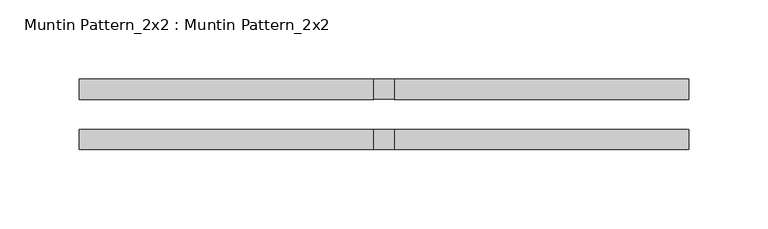
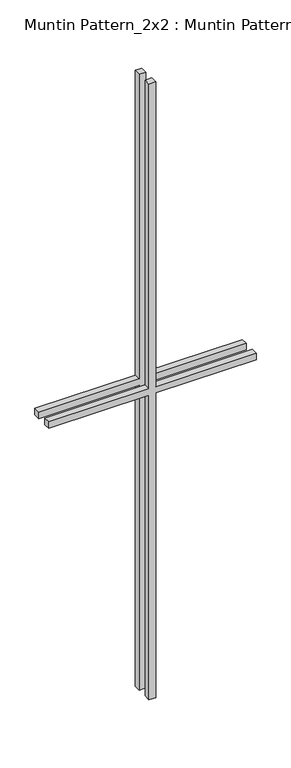
"""IFC4 building model written with IfcOpenShell, lengths in millimetres: proxy geometry, Muntin Pattern_2x2 : Muntin Pattern_2x2."""

import ifcopenshell
import ifcopenshell.guid

model = None  # the IFC model being written
_history = None  # IfcOwnerHistory: only IFC2X3 demands one
_inside = {}  # id of a spatial element -> (the spatial element, [elements in it])
_under = {}  # id of a project, library or spatial element -> (it, [spatial elements below it])
_declared = {}  # id of a project -> (the project, [libraries it declares])
_typed = {}  # id of a type object -> (the type object, [elements of that type])
_made_of = {}  # id of a material, layer set ... -> (it, [elements and type objects made of it])


def new_model(schema):
    """Start an empty IFC model of exactly this schema.

    Asked for "IFC4X3", IfcOpenShell would pick the latest addendum, in which some entities
    have other attributes; the version numbers below select the first issue.
    IFC2X3 requires an IfcOwnerHistory on every rooted entity: one is made here for all.
    """
    global model, _history
    if schema == "IFC4X3":
        model = ifcopenshell.file(schema_version=(4, 3, 0, 0))
    else:
        model = ifcopenshell.file(schema=schema)
    _inside.clear()
    _under.clear()
    _declared.clear()
    _typed.clear()
    _made_of.clear()
    _history = None
    if model.schema == "IFC2X3":
        org = make("IfcOrganization", Name="unknown")
        user = make(
            "IfcPersonAndOrganization",
            ThePerson=make("IfcPerson", FamilyName="unknown"),
            TheOrganization=org,
        )
        app = make(
            "IfcApplication",
            ApplicationDeveloper=org,
            Version="unknown",
            ApplicationFullName="unknown",
            ApplicationIdentifier="unknown",
        )
        _history = make(
            "IfcOwnerHistory",
            OwningUser=user,
            OwningApplication=app,
            ChangeAction="ADDED",
            CreationDate=0,
        )
    return model


def make(cls, **values):
    """One entity of the class cls with the attributes given. An attribute that is None is left unset."""
    return model.create_entity(
        cls, **{name: value for name, value in values.items() if value is not None}
    )


def rooted(cls, **values):
    """An entity with a GlobalId (a new one), such as an element, a storey or a relation."""
    return make(cls, GlobalId=ifcopenshell.guid.new(), OwnerHistory=_history, **values)


def si_unit(unit_type, name, prefix=None):
    """IfcSIUnit, for example si_unit("LENGTHUNIT", "METRE", prefix="MILLI")."""
    return make("IfcSIUnit", UnitType=unit_type, Prefix=prefix, Name=name)


def assignment(units):
    """IfcUnitAssignment: the units of a project."""
    return None if units is None else make("IfcUnitAssignment", Units=units)


def point(xyz):
    """IfcCartesianPoint."""
    return None if xyz is None else make("IfcCartesianPoint", Coordinates=xyz)


def direction(xyz):
    """IfcDirection."""
    return None if xyz is None else make("IfcDirection", DirectionRatios=xyz)


def frame(location, z_axis=None, x_axis=None):
    """IfcAxis2Placement3D, a coordinate frame: its origin and axes. An axis left out is left unset."""
    return make(
        "IfcAxis2Placement3D",
        Location=point(location),
        Axis=direction(z_axis),
        RefDirection=direction(x_axis),
    )


def origin():
    """The frame at (0, 0, 0) with its axes left unset."""
    return frame((0.0, 0.0, 0.0))


def place(relative_to, where):
    """IfcLocalPlacement: puts the frame where relative to a parent placement (None: the world)."""
    return make(
        "IfcLocalPlacement", PlacementRelTo=relative_to, RelativePlacement=where
    )


def context(
    kind, dimensions, precision=None, world=None, true_north=None, identifier=None
):
    """IfcGeometricRepresentationContext, for example the 3D "Model" context."""
    return make(
        "IfcGeometricRepresentationContext",
        ContextIdentifier=identifier,
        ContextType=kind,
        CoordinateSpaceDimension=dimensions,
        Precision=precision,
        WorldCoordinateSystem=world,
        TrueNorth=true_north,
    )


def project(units=None, contexts=None):
    """IfcProject with its units and contexts."""
    return rooted(
        "IfcProject",
        Name="project",
        RepresentationContexts=contexts,
        UnitsInContext=assignment(units),
    )


def spatial(cls, under=None, at=None, **own):
    """A site, building, storey or space (cls), placed at a placement, below another one or the project."""
    s = rooted(cls, ObjectPlacement=at, **own)
    if under is not None:
        _under.setdefault(under.id(), (under, []))[1].append(s)
    return s


def polyline(points):
    """IfcPolyline through the points."""
    return make("IfcPolyline", Points=[point(p) for p in points])


def outline(outer, holes=None, kind="AREA"):
    """IfcArbitraryClosedProfileDef: a profile drawn as a closed curve; with holes, ...WithVoids."""
    if holes is None:
        return make("IfcArbitraryClosedProfileDef", ProfileType=kind, OuterCurve=outer)
    return make(
        "IfcArbitraryProfileDefWithVoids",
        ProfileType=kind,
        OuterCurve=outer,
        InnerCurves=holes,
    )


def extrude(swept, where, along, depth):
    """IfcExtrudedAreaSolid: the profile swept, set in the frame where, extruded along a direction by depth."""
    return make(
        "IfcExtrudedAreaSolid",
        SweptArea=swept,
        Position=where,
        ExtrudedDirection=direction(along),
        Depth=depth,
    )


def shape(context_of_items, identifier, shape_type, items):
    """IfcShapeRepresentation: the items that make up one representation, for example the "Body"."""
    return make(
        "IfcShapeRepresentation",
        ContextOfItems=context_of_items,
        RepresentationIdentifier=identifier,
        RepresentationType=shape_type,
        Items=items,
    )


def source(mapping_origin, context_of_items, identifier, shape_type, items):
    """IfcRepresentationMap: a shape defined once, which mapped items show again and again."""
    return make(
        "IfcRepresentationMap",
        MappingOrigin=mapping_origin,
        MappedRepresentation=shape(context_of_items, identifier, shape_type, items),
    )


def transform(
    local_origin,
    x_axis=None,
    y_axis=None,
    z_axis=None,
    scale=None,
    scale2=None,
    scale3=None,
    uniform=True,
):
    """IfcCartesianTransformationOperator3D, or its non-uniform kind. x_axis, y_axis, z_axis: its Axis1, 2, 3."""
    if uniform:
        return make(
            "IfcCartesianTransformationOperator3D",
            Axis1=direction(x_axis),
            Axis2=direction(y_axis),
            LocalOrigin=point(local_origin),
            Scale=scale,
            Axis3=direction(z_axis),
        )
    return make(
        "IfcCartesianTransformationOperator3DnonUniform",
        Axis1=direction(x_axis),
        Axis2=direction(y_axis),
        LocalOrigin=point(local_origin),
        Scale=scale,
        Axis3=direction(z_axis),
        Scale2=scale2,
        Scale3=scale3,
    )


def mapped(mapping_source, mapping_target):
    """IfcMappedItem: shows the shape of a source again, moved by a transform."""
    return make(
        "IfcMappedItem", MappingSource=mapping_source, MappingTarget=mapping_target
    )


def made_of(thing, what):
    """Note that an element or type object is made of a material, layer set ...; save() writes the relation."""
    if what is not None:
        _made_of.setdefault(what.id(), (what, []))[1].append(thing)
    return thing


def element(
    cls,
    number,
    at=None,
    inside=None,
    cuts=None,
    type_object=None,
    material=None,
    context=None,
    identifier="Body",
    shape_type=None,
    held_by="IfcProductDefinitionShape",
    body=None,
    shapes=None,
    **own,
):
    """One element of the class cls, such as IfcWall. Its Tag is "e" and its number.

    at: its placement. inside: the storey or other place that contains it. cuts: it is an
    opening in that element (IfcRelVoidsElement). A single representation is given by context,
    identifier, shape_type and body (its items); several are given by shapes. held_by: the class
    of the entity that holds the representations. save() writes the other relations.
    """
    e = rooted(cls, Tag="e%d" % number, ObjectPlacement=at, **own)
    if body is not None:
        shapes = [shape(context, identifier, shape_type, body)]
    if shapes is not None:
        e.Representation = make(held_by, Representations=shapes)
    if inside is not None:
        _inside.setdefault(inside.id(), (inside, []))[1].append(e)
    if cuts is not None:
        rooted(
            "IfcRelVoidsElement", RelatingBuildingElement=cuts, RelatedOpeningElement=e
        )
    if type_object is not None:
        _typed.setdefault(type_object.id(), (type_object, []))[1].append(e)
    return made_of(e, material)


def aggregate(whole, parts):
    """IfcRelAggregates: a whole, such as a stair, and the parts it consists of."""
    return rooted("IfcRelAggregates", RelatingObject=whole, RelatedObjects=parts)


def save(model, path):
    """Write the relations noted so far, then the file.

    IfcRelAggregates (storeys below a building ...), IfcRelContainedInSpatialStructure (elements
    in a storey), IfcRelDefinesByType, IfcRelAssociatesMaterial and IfcRelDeclares: one each for
    every whole, place, type object, material and project.
    """
    for whole, parts in _under.values():
        aggregate(whole, parts)
    for where, things in _inside.values():
        rooted(
            "IfcRelContainedInSpatialStructure",
            RelatedElements=things,
            RelatingStructure=where,
        )
    for kind, things in _typed.values():
        rooted("IfcRelDefinesByType", RelatedObjects=things, RelatingType=kind)
    for what, things in _made_of.values():
        rooted("IfcRelAssociatesMaterial", RelatedObjects=things, RelatingMaterial=what)
    for by, libraries in _declared.values():
        rooted("IfcRelDeclares", RelatingContext=by, RelatedDefinitions=libraries)
    model.write(path)


def muntin_pattern_2x2_muntin_pattern_2x2_3dfd0a47(model_context):
    return source(origin(), model_context, "Body", "SweptSolid", [
        extrude(outline(polyline([(609.6, -6.35), (609.6, -192.0875), (596.9, -192.0875), (596.9, -6.35), (0.0, -6.35), (0.0, 6.35), (596.9, 6.35), (596.9, 192.0875), (609.6, 192.0875), (609.6, 6.35), (1206.5, 6.35), (1206.5, -6.35), (609.6, -6.35)])), frame((0.0, -22.225, 0.0), z_axis=(0.0, 1.0, 0.0), x_axis=(0.0, 0.0, 1.0)), (0.0, 0.0, 1.0), 12.7),
        extrude(outline(polyline([(609.6, -6.35), (609.6, -192.0875), (596.9, -192.0875), (596.9, -6.35), (0.0, -6.35), (0.0, 6.35), (596.9, 6.35), (596.9, 192.0875), (609.6, 192.0875), (609.6, 6.35), (1206.5, 6.35), (1206.5, -6.35), (609.6, -6.35)])), frame((0.0, 9.525, 0.0), z_axis=(0.0, 1.0, 0.0), x_axis=(0.0, 0.0, 1.0)), (0.0, 0.0, 1.0), 12.7),
    ])


if __name__ == "__main__":
    model = new_model("IFC4")
    model_context = context("Model", 3, world=origin())
    ifc_project = project(units=[si_unit("LENGTHUNIT", "METRE", prefix="MILLI")], contexts=[model_context])
    site = spatial("IfcSite", under=ifc_project)
    building = spatial("IfcBuilding", under=site)
    placement = place(None, origin())
    muntin_pattern_2x2_muntin_pattern_2x2_shape = muntin_pattern_2x2_muntin_pattern_2x2_3dfd0a47(model_context)
    element("IfcBuildingElementProxy", 1, Name="Muntin Pattern_2x2 : Muntin Pattern_2x2", ObjectType="Muntin Pattern_2x2 : Muntin Pattern_2x2", at=placement, inside=building, context=model_context, shape_type="MappedRepresentation", body=[
        mapped(muntin_pattern_2x2_muntin_pattern_2x2_shape, transform((0.0, 0.0, 0.0), x_axis=(1.0, 0.0, 0.0), y_axis=(0.0, 1.0, 0.0), z_axis=(0.0, 0.0, 1.0))),
    ])
    save(model, "model.ifc")

# Revit data of these elements
# Type "Muntin Pattern_2x2 : Muntin Pattern_2x2"
#   Width [instance default] = 4' - 0"
#   Thickness = 0' - 0 1/2"
#   Height [instance default] = 4' - 0"
#   Distance = 0' - 0 3/4"
#   Interior Material [instance default] = none
#   Exterior Material [instance default] = none
#   Default Elevation = 0
# Element 1 (IfcBuildingElementProxy, "Muntin Pattern_2x2 : Muntin Pattern_2x2")
#   Width = 1' - 3 1/8"
#   Height = 3' - 11 1/2"
#   Interior Material = Wood - Stained
#   Exterior Material = Clad - White
#   Materials on its faces: "Clad - White", "Wood - Stained"
# Materials
#   "Clad - White": class "Wood", colour RGB 216 216 204, transparency 0, Cost = 0
#   "Wood - Stained": class "Wood", colour RGB 224 178 126, transparency 0, Cost = 0
